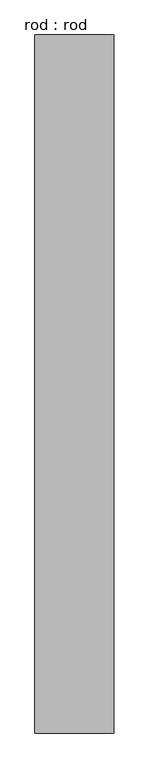
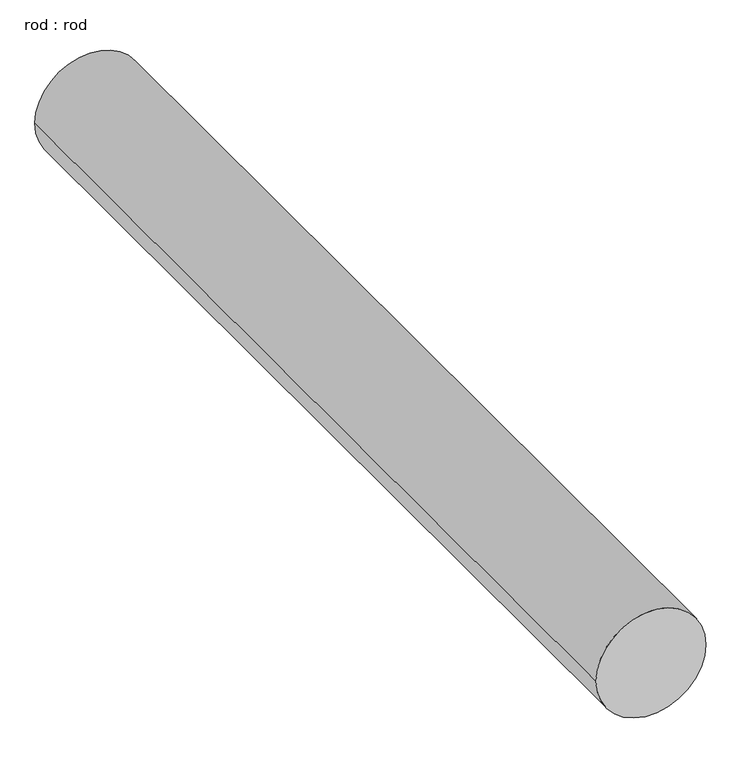
"""IFC4 building model written with IfcOpenShell, lengths in millimetres: proxy geometry, rod : rod."""

from ifc_helpers import new_model, si_unit, point, frame, frame_2d, origin, place, context, project, spatial, circle_curve, trimmed, segment, composite_curve, outline, extrude, source, transform, mapped, element, save


def rod_rod_fedebc19(model_context):
    return source(origin(), model_context, "Body", "SweptSolid", [
        extrude(outline(composite_curve([segment(trimmed(circle_curve(frame_2d((0.0108462, 0.0)), 200.0), [point((0.0108462, 200.0))], [point((0.0108462, -200.0))], False, "CARTESIAN"), True, "CONTINUOUS"), segment(trimmed(circle_curve(frame_2d((0.0108462, 0.0)), 200.0), [point((0.0108462, -200.0))], [point((0.0108462, 200.0))], False, "CARTESIAN"), True, "CONTINUOUS")], self_intersect=False)), frame((0.0, 2322.7286153, 0.0), z_axis=(0.0, 1.0, 0.0), x_axis=(0.0, 0.0, 1.0)), (0.0, 0.0, 1.0), 3540.0),
    ])


if __name__ == "__main__":
    model = new_model("IFC4")
    model_context = context("Model", 3, world=origin())
    ifc_project = project(units=[si_unit("LENGTHUNIT", "METRE", prefix="MILLI")], contexts=[model_context])
    site = spatial("IfcSite", under=ifc_project)
    building = spatial("IfcBuilding", under=site)
    placement = place(None, origin())
    rod_rod_shape = rod_rod_fedebc19(model_context)
    element("IfcBuildingElementProxy", 1, Name="rod : rod", ObjectType="rod : rod", at=placement, inside=building, context=model_context, shape_type="MappedRepresentation", body=[
        mapped(rod_rod_shape, transform((0.0, 0.0, 0.0), x_axis=(1.0, 0.0, 0.0), y_axis=(0.0, 1.0, 0.0), z_axis=(0.0, 0.0, 1.0))),
    ])
    save(model, "model.ifc")

# Revit data of these elements
# Type "rod : rod"
#   Default Elevation = 0
